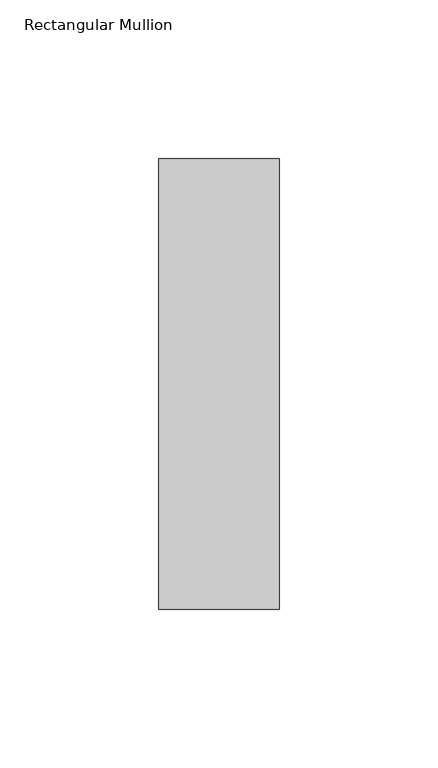
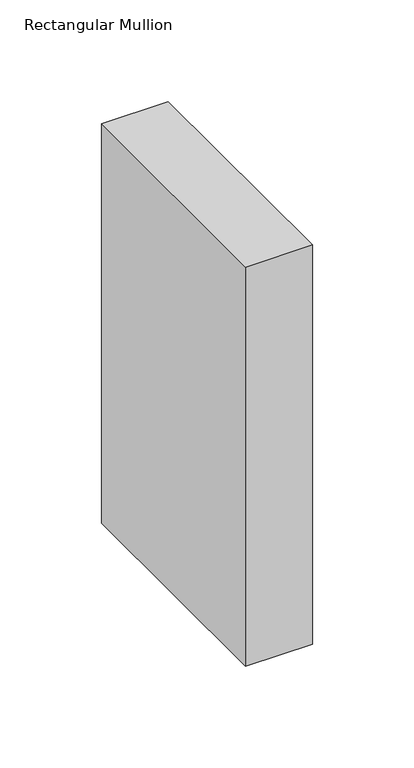
"""IFC4 building model written with IfcOpenShell, lengths in millimetres: member geometry, Rectangular Mullion : NLRS_21_CWM_hsb-regel 38x142_gen_rsf."""

from ifc_helpers import new_model, si_unit, frame, origin, place, context, project, spatial, polyline, outline, extrude, source, transform, mapped, element, save


def rectangular_mullion_e6972d68(model_context):
    return source(origin(), model_context, "Body", "SweptSolid", [
        extrude(outline(polyline([(0.0, -71.0), (-38.0, -71.0), (-38.0, 71.0), (0.0, 71.0), (0.0, -71.0)])), frame((0.0, 0.0, -239.8441061), z_axis=(0.0, 0.0, 1.0), x_axis=(1.0, 0.0, 0.0)), (0.0, 0.0, 1.0), 239.8441061),
    ])


if __name__ == "__main__":
    model = new_model("IFC4")
    model_context = context("Model", 3, world=origin())
    ifc_project = project(units=[si_unit("LENGTHUNIT", "METRE", prefix="MILLI")], contexts=[model_context])
    site = spatial("IfcSite", under=ifc_project)
    building = spatial("IfcBuilding", under=site)
    placement = place(None, origin())
    rectangular_mullion_shape = rectangular_mullion_e6972d68(model_context)
    element("IfcMember", 1, ObjectType="Rectangular Mullion : NLRS_21_CWM_hsb-regel 38x142_gen_rsf", at=placement, inside=building, context=model_context, shape_type="MappedRepresentation", body=[
        mapped(rectangular_mullion_shape, transform((0.0, 0.0, 0.0), x_axis=(1.0, 0.0, 0.0), y_axis=(0.0, 1.0, 0.0), z_axis=(0.0, 0.0, 1.0))),
    ])
    save(model, "model.ifc")

# Revit data of these elements
# Type "Rectangular Mullion : NLRS_21_CWM_hsb-regel 38x142_gen_rsf"
#   Export Type to IFC As = "IfcWall"
#   Type IfcGUID = "07M7mRoiH1CR8m_RSKIwpF"
#   Assembly Code = "21.10"
#   built-in parameter 1007322 = 0.465879 (stored number, unit not read)
#   built-in parameter 1007321 = 0.062336 (stored number, unit not read)
#   built-in parameter 1007320 = 0.062336 (stored number, unit not read)
# Element 1 (IfcMember, "Rectangular Mullion : NLRS_21_CWM_hsb-regel 38x142_gen_rsf")
#   Materials on its faces: "NLRS_i2_hout naaldhout vuren_gen_rsf"
# Materials
#   "NLRS_i2_hout naaldhout vuren_gen_rsf": class "I - Hout", colour RGB 234 199 147, transparency 0, Keynote = "i2", Manufacturer = "Revit Standards Foundation", URL = "www.revitstandards.org", Description = "hout vuren", Cost = 0
